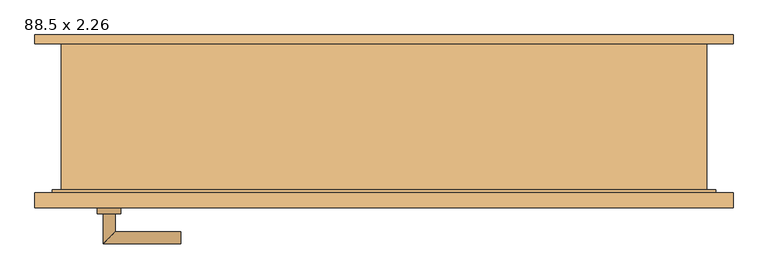
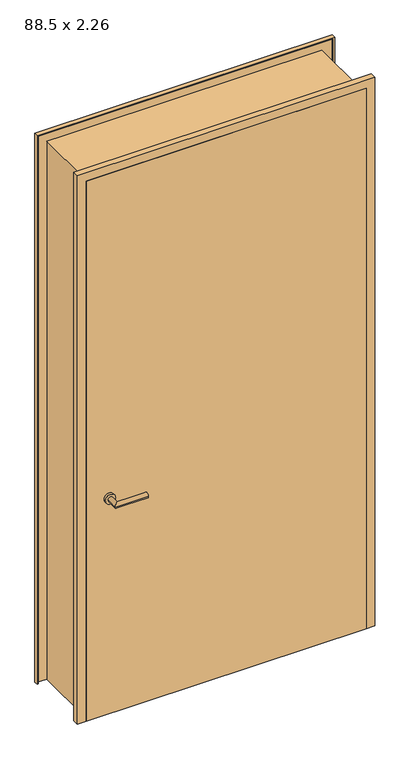
"""IFC4 building model written with IfcOpenShell, lengths in millimetres: door geometry, Drehflügel 1-flg - Stahlzarge : 88.5 x 2.26."""

from ifc_helpers import new_model, si_unit, point, frame, frame_2d, origin, place, context, project, spatial, polyline, circle_curve, ellipse_curve, trimmed, segment, composite_curve, outline, extrude, faceted_brep, source, transform, mapped, element, save
from ifc_brep_helpers import plane_surface, cylinder_surface, advanced_brep


def door_88_5_x_2_26_a3dffa5d(model_context):
    return source(origin(), model_context, "Body", "SolidModel", [
        advanced_brep(
        [(-471.4, -114.4346141, 1000.0), (-451.4, -114.4346141, 1000.0), (-451.4, -64.4346141, 1000.0), (-471.4, -44.4346141, 1000.0), (-341.4, -44.4346141, 1000.0), (-341.4, -64.4346141, 1000.0)],
        [
            (0, 1, circle_curve(frame((-461.4, -114.4346141, 1000.0), z_axis=(0.0, -1.0, 0.0), x_axis=(1.0, 0.0, 0.0)), 10.0)),
            (1, 0, circle_curve(frame((-461.4, -114.4346141, 1000.0), z_axis=(0.0, -1.0, 0.0), x_axis=(1.0, 0.0, 0.0)), 10.0)),
            (1, 2),
            (2, 3, ellipse_curve(frame((-461.4, -54.4346141, 1000.0), z_axis=(-0.7071067811865385, -0.7071067811865565, 0.0), x_axis=(0.7071067811865563, -0.7071067811865386, 0.0)), 14.1421356, 10.0)),
            (3, 0),
            (3, 2, ellipse_curve(frame((-461.4, -54.4346141, 1000.0), z_axis=(-0.7071067811865385, -0.7071067811865565, 0.0), x_axis=(0.7071067811865563, -0.7071067811865386, 0.0)), 14.1421356, 10.0)),
            (4, 5, circle_curve(frame((-341.4, -54.4346141, 1000.0), z_axis=(1.0, 0.0, 0.0), x_axis=(0.0, -1.0, 0.0)), 10.0)),
            (5, 4, circle_curve(frame((-341.4, -54.4346141, 1000.0), z_axis=(1.0, 0.0, 0.0), x_axis=(0.0, -1.0, 0.0)), 10.0)),
            (2, 5),
            (4, 3),
        ],
        [
            plane_surface(frame((-461.4, -114.4346141, -287.7526403), z_axis=(0.0, -1.0, 0.0), x_axis=(0.0, 0.0, 1.0))),
            cylinder_surface(frame((-461.4, -114.4346141, 1000.0), z_axis=(0.0, -1.0, 0.0), x_axis=(1.0, 0.0, 0.0)), 10.0),
            plane_surface(frame((-341.4, -54.4346141, -287.7526403), z_axis=(1.0, 0.0, 0.0), x_axis=(0.0, 0.0, 1.0))),
            cylinder_surface(frame((-461.4, -54.4346141, 1000.0), z_axis=(-1.0, 0.0, 0.0), x_axis=(0.0, -1.0, 0.0)), 10.0),
        ],
        [
            (0, [[1, 2]]),
            (1, [[3, 4, 5, -2]]),
            (1, [[-5, 6, -3, -1]]),
            (2, [[7, 8]]),
            (3, [[9, -7, 10, -4]]),
            (3, [[-10, -8, -9, -6]]),
        ],
    ),
        advanced_brep(
        [(-451.4, -174.4346141, 1000.0), (-471.4, -174.4346141, 1000.0), (-471.4, -224.4346141, 1000.0), (-451.4, -204.4346141, 1000.0), (-341.4, -204.4346141, 1000.0), (-341.4, -224.4346141, 1000.0)],
        [
            (0, 1, circle_curve(frame((-461.4, -174.4346141, 1000.0), z_axis=(0.0, 1.0, 0.0), x_axis=(-1.0, 0.0, 0.0)), 10.0)),
            (1, 0, circle_curve(frame((-461.4, -174.4346141, 1000.0), z_axis=(0.0, 1.0, 0.0), x_axis=(-1.0, 0.0, 0.0)), 10.0)),
            (1, 2),
            (2, 3, ellipse_curve(frame((-461.4, -214.4346141, 1000.0), z_axis=(-0.7071067811865475, 0.7071067811865475, 0.0), x_axis=(0.7071067811865474, 0.7071067811865476, 0.0)), 14.1421356, 10.0)),
            (3, 0),
            (3, 2, ellipse_curve(frame((-461.4, -214.4346141, 1000.0), z_axis=(-0.7071067811865475, 0.7071067811865475, 0.0), x_axis=(0.7071067811865474, 0.7071067811865476, 0.0)), 14.1421356, 10.0)),
            (4, 5, circle_curve(frame((-341.4, -214.4346141, 1000.0), z_axis=(1.0, 0.0, 0.0), x_axis=(0.0, -1.0, 0.0)), 10.0)),
            (5, 4, circle_curve(frame((-341.4, -214.4346141, 1000.0), z_axis=(1.0, 0.0, 0.0), x_axis=(0.0, -1.0, 0.0)), 10.0)),
            (2, 5),
            (4, 3),
        ],
        [
            plane_surface(frame((-461.4, -174.4346141, -287.7526403), z_axis=(0.0, 1.0, 0.0), x_axis=(0.0, 0.0, 1.0))),
            cylinder_surface(frame((-461.4, -174.4346141, 1000.0), z_axis=(0.0, 1.0, 0.0), x_axis=(-1.0, 0.0, 0.0)), 10.0),
            plane_surface(frame((-341.4, -214.4346141, -287.7526403), z_axis=(1.0, 0.0, 0.0), x_axis=(0.0, 0.0, 1.0))),
            cylinder_surface(frame((-461.4, -214.4346141, 1000.0), z_axis=(-1.0, 0.0, 0.0), x_axis=(0.0, -1.0, 0.0)), 10.0),
        ],
        [
            (0, [[1, 2]]),
            (1, [[3, 4, 5, -2]]),
            (1, [[-5, 6, -3, -1]]),
            (2, [[7, 8]]),
            (3, [[9, -7, 10, -4]]),
            (3, [[-10, -8, -9, -6]]),
        ],
    ),
        extrude(outline(composite_curve([segment(trimmed(circle_curve(frame_2d((1000.0, -461.4)), 20.0), [point((1000.0, -481.4))], [point((1000.0, -441.4))], False, "CARTESIAN"), True, "CONTINUOUS"), segment(trimmed(circle_curve(frame_2d((1000.0, -461.4)), 20.0), [point((1000.0, -441.4))], [point((1000.0, -481.4))], False, "CARTESIAN"), True, "CONTINUOUS")], self_intersect=False)), frame((0.0, -114.4346141, 0.0), z_axis=(0.0, 1.0, 0.0), x_axis=(0.0, 0.0, 1.0)), (0.0, 0.0, 1.0), 10.0),
        extrude(outline(composite_curve([segment(trimmed(circle_curve(frame_2d((1000.0, -461.4)), 20.0), [point((1000.0, -481.4))], [point((1000.0, -441.4))], False, "CARTESIAN"), True, "CONTINUOUS"), segment(trimmed(circle_curve(frame_2d((1000.0, -461.4)), 20.0), [point((1000.0, -441.4))], [point((1000.0, -481.4))], False, "CARTESIAN"), True, "CONTINUOUS")], self_intersect=False)), frame((0.0, -174.4346141, 0.0), z_axis=(0.0, 1.0, 0.0), x_axis=(0.0, 0.0, 1.0)), (0.0, 0.0, 1.0), 10.0),
        extrude(outline(polyline([(551.4, -139.4346141), (551.4, -164.4346141), (-551.4, -164.4346141), (-551.4, -139.4346141), (551.4, -139.4346141)])), frame((0.0, 0.0, 100.0), z_axis=(0.0, 0.0, 1.0), x_axis=(1.0, 0.0, 0.0)), (0.0, 0.0, 1.0), 2250.0),
        faceted_brep([(585.8603207, 125.5653859, 100.0), (585.8603207, 110.5653859, 100.0), (580.8603207, 110.5653859, 100.0), (580.8603207, 120.5653859, 100.0), (541.4, 120.5653859, 100.0), (541.4, -134.4346141, 100.0), (556.4, -134.4346141, 100.0), (556.4, -159.4346141, 100.0), (580.8603207, -159.4346141, 100.0), (580.8603207, -139.4346141, 100.0), (585.8603207, -139.4346141, 100.0), (585.8603207, -164.4346141, 100.0), (551.4, -164.4346141, 100.0), (551.4, -139.4346141, 100.0), (536.4, -139.4346141, 100.0), (536.4, 125.5653859, 100.0), (536.4, 125.5653859, 2335.0), (-536.4, 125.5653859, 2335.0), (-536.4, 125.5653859, 100.0), (-585.8603207, 125.5653859, 100.0), (-585.8603207, 125.5653859, 2384.4603207), (585.8603207, 125.5653859, 2384.4603207), (536.4, -139.4346141, 2335.0), (551.4, -139.4346141, 2350.0), (-551.4, -139.4346141, 2350.0), (-551.4, -139.4346141, 100.0), (-536.4, -139.4346141, 100.0), (-536.4, -139.4346141, 2335.0), (551.4, -164.4346141, 2350.0), (585.8603207, -164.4346141, 2384.4603207), (-585.8603207, -164.4346141, 2384.4603207), (-585.8603207, -164.4346141, 100.0), (-551.4, -164.4346141, 100.0), (-551.4, -164.4346141, 2350.0), (585.8603207, -139.4346141, 2384.4603207), (580.8603207, -139.4346141, 2379.4603207), (-580.8603207, -139.4346141, 2379.4603207), (-580.8603207, -139.4346141, 100.0), (-585.8603207, -139.4346141, 100.0), (-585.8603207, -139.4346141, 2384.4603207), (580.8603207, -159.4346141, 2379.4603207), (556.4, -159.4346141, 2355.0), (-556.4, -159.4346141, 2355.0), (-556.4, -159.4346141, 100.0), (-580.8603207, -159.4346141, 100.0), (-580.8603207, -159.4346141, 2379.4603207), (556.4, -134.4346141, 2355.0), (541.4, -134.4346141, 2340.0), (-541.4, -134.4346141, 2340.0), (-541.4, -134.4346141, 100.0), (-556.4, -134.4346141, 100.0), (-556.4, -134.4346141, 2355.0), (541.4, 120.5653859, 2340.0), (580.8603207, 120.5653859, 2379.4603207), (-580.8603207, 120.5653859, 2379.4603207), (-580.8603207, 120.5653859, 100.0), (-541.4, 120.5653859, 100.0), (-541.4, 120.5653859, 2340.0), (580.8603207, 110.5653859, 2379.4603207), (585.8603207, 110.5653859, 2384.4603207), (-585.8603207, 110.5653859, 2384.4603207), (-585.8603207, 110.5653859, 100.0), (-580.8603207, 110.5653859, 100.0), (-580.8603207, 110.5653859, 2379.4603207)], [[[0, 1, 2, 3, 4, 5, 6, 7, 8, 9, 10, 11, 12, 13, 14, 15]], [[15, 16, 17, 18, 19, 20, 21, 0]], [[14, 22, 16, 15]], [[13, 23, 24, 25, 26, 27, 22, 14]], [[12, 28, 23, 13]], [[11, 29, 30, 31, 32, 33, 28, 12]], [[10, 34, 29, 11]], [[9, 35, 36, 37, 38, 39, 34, 10]], [[8, 40, 35, 9]], [[7, 41, 42, 43, 44, 45, 40, 8]], [[6, 46, 41, 7]], [[5, 47, 48, 49, 50, 51, 46, 6]], [[4, 52, 47, 5]], [[3, 53, 54, 55, 56, 57, 52, 4]], [[2, 58, 53, 3]], [[1, 59, 60, 61, 62, 63, 58, 2]], [[0, 21, 59, 1]], [[20, 19, 61, 60]], [[19, 18, 26, 25, 32, 31, 38, 37, 44, 43, 50, 49, 56, 55, 62, 61]], [[27, 26, 18, 17]], [[33, 32, 25, 24]], [[39, 38, 31, 30]], [[45, 44, 37, 36]], [[51, 50, 43, 42]], [[57, 56, 49, 48]], [[63, 62, 55, 54]], [[22, 27, 17, 16]], [[28, 33, 24, 23]], [[34, 39, 30, 29]], [[40, 45, 36, 35]], [[46, 51, 42, 41]], [[52, 57, 48, 47]], [[58, 63, 54, 53]], [[21, 20, 60, 59]]]),
    ])


if __name__ == "__main__":
    model = new_model("IFC4")
    model_context = context("Model", 3, world=origin())
    ifc_project = project(units=[si_unit("LENGTHUNIT", "METRE", prefix="MILLI")], contexts=[model_context])
    site = spatial("IfcSite", under=ifc_project)
    building = spatial("IfcBuilding", under=site)
    placement = place(None, origin())
    door_88_5_x_2_26_shape = door_88_5_x_2_26_a3dffa5d(model_context)
    element("IfcDoor", 1, ObjectType="Drehflügel 1-flg - Stahlzarge : 88.5 x 2.26", at=placement, inside=building, context=model_context, shape_type="MappedRepresentation", body=[
        mapped(door_88_5_x_2_26_shape, transform((0.0, 0.0, 0.0), x_axis=(1.0, 0.0, 0.0), y_axis=(0.0, 1.0, 0.0), z_axis=(0.0, 0.0, 1.0))),
    ])
    save(model, "model.ifc")

# Revit data of these elements
# Type "Drehflügel 1-flg - Stahlzarge : 88.5 x 2.26"
#   Construction Type Id = "MDOOR"
#   Type Mark = "20"
#   Operation = "SingleSwingRight"
#   Keynote = "16.03"
#   Analytic Construction = "Metall"
#   Thermal Resistance (R) = 0.270117 (m²·K)/W
#   Heat Transfer Coefficient (U) = 3.7021 W/(m²·K)
#   Rough Width = 1.1228 m
#   Rough Height [instance default] = 2.360 m
#   Höhe Türgriff [instance default] = 0.900 m
#   Height = 2.260 m
#   Fußbodenaufbau [instance default] = 0.100 m
#   Width = 1.1228 m
#   Sichtbarkeit Sturzlinien [instance default] = yes
#   Türgriff auswählen [instance default] = element 221079
#   Türgriff [instance default] = none
#   Türflügel [instance default] = none
#   Rahmen/Pfosten [instance default] = Metall - Lackiert - Grau
#   Visual Light Transmittance = 0
#   Solar Heat Gain Coefficient = 0
#   Function = (empty or 0)
#   Wall Closure = (empty or 0)
# Element 1 (IfcDoor, "Drehflügel 1-flg - Stahlzarge : 88.5 x 2.26")
#   Materials on its faces: "Metall - Lackiert - Grau", "Metall - Chrom", "Holz - Birke"
# Materials
#   "Metall - Lackiert - Grau": class "Farbe 1", colour RGB 98 98 98, transparency 0, Cost = 0
#   "Metall - Chrom": class "Metall", colour RGB 247 247 247, transparency 0, Cost = 0
#   "Holz - Birke": class "Holz", colour RGB 213 164 103, transparency 0, Cost = 0
